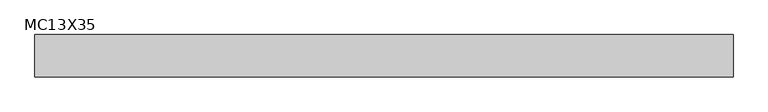
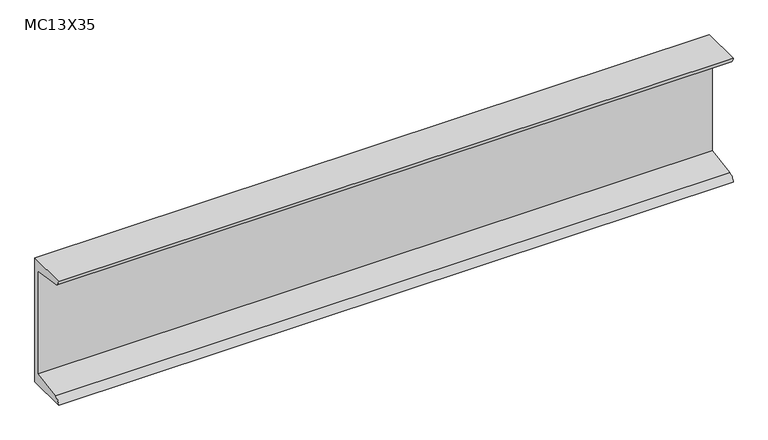
"""IFC4 building model written with IfcOpenShell, lengths in millimetres: beam geometry, MC-Miscellaneous Channel : MC13X35."""

from ifc_helpers import new_model, si_unit, point, frame, frame_2d, origin, place, context, project, spatial, polyline, circle_curve, trimmed, segment, composite_curve, outline, extrude, source, transform, mapped, element, save


def mc13x35_ec1bf522(model_context):
    return source(origin(), model_context, "Body", "SweptSolid", [
        extrude(outline(composite_curve([segment(polyline([(24.892, 165.1), (24.892, -165.1), (-78.486, -165.1)]), True, "CONTINUOUS"), segment(trimmed(circle_curve(frame_2d((-62.992, -165.1)), 15.494), [point((-78.486, -165.1))], [point((-62.992, -149.606))], False, "CARTESIAN"), True, "CONTINUOUS"), segment(polyline([(-62.992, -149.606), (13.5382, -137.4848071), (13.5382, 137.4848071), (-62.992, 149.606)]), True, "CONTINUOUS"), segment(trimmed(circle_curve(frame_2d((-62.992, 165.1)), 15.494), [point((-62.992, 149.606))], [point((-78.486, 165.1))], False, "CARTESIAN"), True, "CONTINUOUS"), segment(polyline([(-78.486, 165.1), (24.892, 165.1)]), True, "CONTINUOUS")], self_intersect=False)), frame((-850.9, 0.0, 0.0), z_axis=(1.0, 0.0, 0.0), x_axis=(0.0, 1.0, 0.0)), (0.0, 0.0, 1.0), 1701.8),
    ])


if __name__ == "__main__":
    model = new_model("IFC4")
    model_context = context("Model", 3, world=origin())
    ifc_project = project(units=[si_unit("LENGTHUNIT", "METRE", prefix="MILLI")], contexts=[model_context])
    site = spatial("IfcSite", under=ifc_project)
    building = spatial("IfcBuilding", under=site)
    placement = place(None, origin())
    mc13x35_shape = mc13x35_ec1bf522(model_context)
    element("IfcBeam", 1, ObjectType="MC-Miscellaneous Channel : MC13X35", at=placement, inside=building, context=model_context, shape_type="MappedRepresentation", body=[
        mapped(mc13x35_shape, transform((0.0, 0.0, 0.0), x_axis=(1.0, 0.0, 0.0), y_axis=(0.0, 1.0, 0.0), z_axis=(0.0, 0.0, 1.0))),
    ])
    save(model, "model.ifc")

# Revit data of these elements
# Type "MC-Miscellaneous Channel : MC13X35"
#   Assembly Code = "B10"
#   W = 35
#   Length [instance default] = 5' - 0"
#   bf = 0' - 4.07"
#   d = 1' - 1"
#   tf = 0' - 0.61"
#   tw = 0' - 0.447"
#   x = 0' - 0.98"
#   A = 0.0715278 SF
#   Structural Material [instance default] = Steel ASTM A36
# Element 1 (IfcBeam, "MC-Miscellaneous Channel : MC13X35")
#   Structural Material = Steel ASTM A992
#   Materials on its faces: "Steel ASTM A992"
# Materials
#   "Steel ASTM A36": class "Metal", colour RGB 199 199 199, transparency 0, Description = "Structural steel, ASTM A36 Grade B, mill finish", Cost = 0
#   "Steel ASTM A992": class "Metal", colour RGB 199 199 199, transparency 0, Description = "Structural steel 50ksi", Cost = 0
